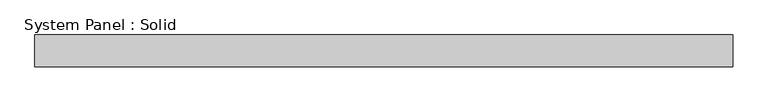
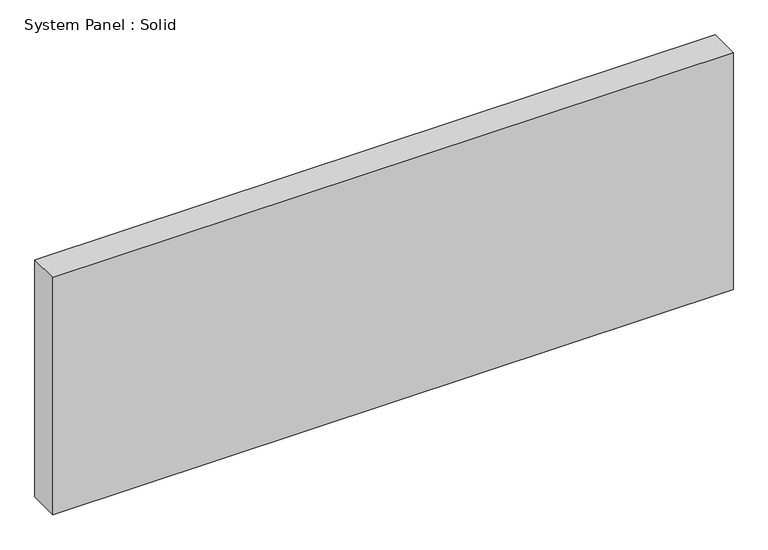
"""IFC4 building model written with IfcOpenShell, lengths in millimetres: plate geometry, System Panel : Solid."""

from ifc_helpers import new_model, si_unit, origin, origin_with_axes, place, context, project, spatial, polyline, outline, extrude, source, transform, mapped, element, save


def system_panel_solid_21827ae2(model_context):
    return source(origin(), model_context, "Body", "SweptSolid", [
        extrude(outline(polyline([(697.4416668, -19.05), (-697.4416668, -19.05), (-697.4416668, 44.45), (697.4416668, 44.45), (697.4416668, -19.05)])), origin_with_axes(), (0.0, 0.0, 1.0), 514.35),
    ])


if __name__ == "__main__":
    model = new_model("IFC4")
    model_context = context("Model", 3, world=origin())
    ifc_project = project(units=[si_unit("LENGTHUNIT", "METRE", prefix="MILLI")], contexts=[model_context])
    site = spatial("IfcSite", under=ifc_project)
    building = spatial("IfcBuilding", under=site)
    placement = place(None, origin())
    system_panel_solid_shape = system_panel_solid_21827ae2(model_context)
    element("IfcPlate", 1, ObjectType="System Panel : Solid", at=placement, inside=building, context=model_context, shape_type="MappedRepresentation", body=[
        mapped(system_panel_solid_shape, transform((0.0, 0.0, 0.0), x_axis=(1.0, 0.0, 0.0), y_axis=(0.0, 1.0, 0.0), z_axis=(0.0, 0.0, 1.0))),
    ])
    save(model, "model.ifc")

# Revit data of these elements
# Type "System Panel : Solid"
#   Construction Type Id = "MDOOR"
#   Analytic Construction = "Metal"
#   Visual Light Transmittance = 0
#   Solar Heat Gain Coefficient = 0
#   Heat Transfer Coefficient (U) = 0.651978 BTU/(h·ft²·°F)
#   Define Thermal Properties by = 1
# Element 1 (IfcPlate, "System Panel : Solid")
#   Materials on its faces: "Default"
# Materials
#   "Default": class "Miscellaneous", colour RGB 127 127 127, transparency 0, Cost = 0
